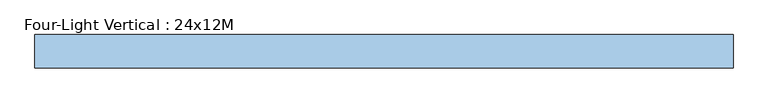
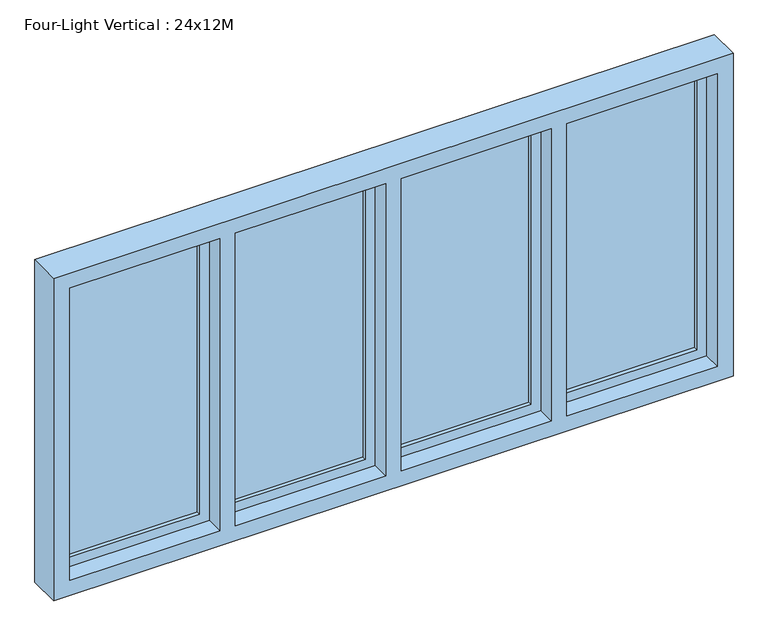
"""IFC4 building model written with IfcOpenShell, lengths in millimetres: window geometry, Four-Light Vertical : 24x12M."""

import ifcopenshell
import ifcopenshell.guid

model = None  # the IFC model being written
_history = None  # IfcOwnerHistory: only IFC2X3 demands one
_inside = {}  # id of a spatial element -> (the spatial element, [elements in it])
_under = {}  # id of a project, library or spatial element -> (it, [spatial elements below it])
_declared = {}  # id of a project -> (the project, [libraries it declares])
_typed = {}  # id of a type object -> (the type object, [elements of that type])
_made_of = {}  # id of a material, layer set ... -> (it, [elements and type objects made of it])


def new_model(schema):
    """Start an empty IFC model of exactly this schema.

    Asked for "IFC4X3", IfcOpenShell would pick the latest addendum, in which some entities
    have other attributes; the version numbers below select the first issue.
    IFC2X3 requires an IfcOwnerHistory on every rooted entity: one is made here for all.
    """
    global model, _history
    if schema == "IFC4X3":
        model = ifcopenshell.file(schema_version=(4, 3, 0, 0))
    else:
        model = ifcopenshell.file(schema=schema)
    _inside.clear()
    _under.clear()
    _declared.clear()
    _typed.clear()
    _made_of.clear()
    _history = None
    if model.schema == "IFC2X3":
        org = make("IfcOrganization", Name="unknown")
        user = make(
            "IfcPersonAndOrganization",
            ThePerson=make("IfcPerson", FamilyName="unknown"),
            TheOrganization=org,
        )
        app = make(
            "IfcApplication",
            ApplicationDeveloper=org,
            Version="unknown",
            ApplicationFullName="unknown",
            ApplicationIdentifier="unknown",
        )
        _history = make(
            "IfcOwnerHistory",
            OwningUser=user,
            OwningApplication=app,
            ChangeAction="ADDED",
            CreationDate=0,
        )
    return model


def make(cls, **values):
    """One entity of the class cls with the attributes given. An attribute that is None is left unset."""
    return model.create_entity(
        cls, **{name: value for name, value in values.items() if value is not None}
    )


def rooted(cls, **values):
    """An entity with a GlobalId (a new one), such as an element, a storey or a relation."""
    return make(cls, GlobalId=ifcopenshell.guid.new(), OwnerHistory=_history, **values)


def si_unit(unit_type, name, prefix=None):
    """IfcSIUnit, for example si_unit("LENGTHUNIT", "METRE", prefix="MILLI")."""
    return make("IfcSIUnit", UnitType=unit_type, Prefix=prefix, Name=name)


def assignment(units):
    """IfcUnitAssignment: the units of a project."""
    return None if units is None else make("IfcUnitAssignment", Units=units)


def point(xyz):
    """IfcCartesianPoint."""
    return None if xyz is None else make("IfcCartesianPoint", Coordinates=xyz)


def direction(xyz):
    """IfcDirection."""
    return None if xyz is None else make("IfcDirection", DirectionRatios=xyz)


def frame(location, z_axis=None, x_axis=None):
    """IfcAxis2Placement3D, a coordinate frame: its origin and axes. An axis left out is left unset."""
    return make(
        "IfcAxis2Placement3D",
        Location=point(location),
        Axis=direction(z_axis),
        RefDirection=direction(x_axis),
    )


def origin():
    """The frame at (0, 0, 0) with its axes left unset."""
    return frame((0.0, 0.0, 0.0))


def place(relative_to, where):
    """IfcLocalPlacement: puts the frame where relative to a parent placement (None: the world)."""
    return make(
        "IfcLocalPlacement", PlacementRelTo=relative_to, RelativePlacement=where
    )


def context(
    kind, dimensions, precision=None, world=None, true_north=None, identifier=None
):
    """IfcGeometricRepresentationContext, for example the 3D "Model" context."""
    return make(
        "IfcGeometricRepresentationContext",
        ContextIdentifier=identifier,
        ContextType=kind,
        CoordinateSpaceDimension=dimensions,
        Precision=precision,
        WorldCoordinateSystem=world,
        TrueNorth=true_north,
    )


def project(units=None, contexts=None):
    """IfcProject with its units and contexts."""
    return rooted(
        "IfcProject",
        Name="project",
        RepresentationContexts=contexts,
        UnitsInContext=assignment(units),
    )


def spatial(cls, under=None, at=None, **own):
    """A site, building, storey or space (cls), placed at a placement, below another one or the project."""
    s = rooted(cls, ObjectPlacement=at, **own)
    if under is not None:
        _under.setdefault(under.id(), (under, []))[1].append(s)
    return s


def polyline(points):
    """IfcPolyline through the points."""
    return make("IfcPolyline", Points=[point(p) for p in points])


def outline(outer, holes=None, kind="AREA"):
    """IfcArbitraryClosedProfileDef: a profile drawn as a closed curve; with holes, ...WithVoids."""
    if holes is None:
        return make("IfcArbitraryClosedProfileDef", ProfileType=kind, OuterCurve=outer)
    return make(
        "IfcArbitraryProfileDefWithVoids",
        ProfileType=kind,
        OuterCurve=outer,
        InnerCurves=holes,
    )


def extrude(swept, where, along, depth):
    """IfcExtrudedAreaSolid: the profile swept, set in the frame where, extruded along a direction by depth."""
    return make(
        "IfcExtrudedAreaSolid",
        SweptArea=swept,
        Position=where,
        ExtrudedDirection=direction(along),
        Depth=depth,
    )


def faces_of(points, faces, orient=None, outer=None):
    """IfcFace entities. A face is a list of loops; a loop is a list of indices into points, from 0.

    orient and outer hold one flag for each loop. By default every Orientation is true, the
    first loop of a face is its IfcFaceOuterBound and the others are IfcFaceBound.
    """
    made = []
    for i, loops in enumerate(faces):
        bounds = []
        for j, loop in enumerate(loops):
            is_outer = j == 0 if outer is None else outer[i][j]
            bounds.append(
                make(
                    "IfcFaceOuterBound" if is_outer else "IfcFaceBound",
                    Bound=make("IfcPolyLoop", Polygon=[points[k] for k in loop]),
                    Orientation=True if orient is None else orient[i][j],
                )
            )
        made.append(make("IfcFace", Bounds=bounds))
    return made


def faceted_brep(points, faces, orient=None, outer=None, voids=None):
    """IfcFacetedBrep: a solid bounded by flat faces; with voids (closed shells), ...WithVoids."""
    shared = [point(p) for p in points]
    hull = make("IfcClosedShell", CfsFaces=faces_of(shared, faces, orient, outer))
    if voids is None:
        return make("IfcFacetedBrep", Outer=hull)
    return make(
        "IfcFacetedBrepWithVoids",
        Outer=hull,
        Voids=[
            make(cls, CfsFaces=faces_of(shared, fs, o, b)) for cls, fs, o, b in voids
        ],
    )


def shape(context_of_items, identifier, shape_type, items):
    """IfcShapeRepresentation: the items that make up one representation, for example the "Body"."""
    return make(
        "IfcShapeRepresentation",
        ContextOfItems=context_of_items,
        RepresentationIdentifier=identifier,
        RepresentationType=shape_type,
        Items=items,
    )


def source(mapping_origin, context_of_items, identifier, shape_type, items):
    """IfcRepresentationMap: a shape defined once, which mapped items show again and again."""
    return make(
        "IfcRepresentationMap",
        MappingOrigin=mapping_origin,
        MappedRepresentation=shape(context_of_items, identifier, shape_type, items),
    )


def transform(
    local_origin,
    x_axis=None,
    y_axis=None,
    z_axis=None,
    scale=None,
    scale2=None,
    scale3=None,
    uniform=True,
):
    """IfcCartesianTransformationOperator3D, or its non-uniform kind. x_axis, y_axis, z_axis: its Axis1, 2, 3."""
    if uniform:
        return make(
            "IfcCartesianTransformationOperator3D",
            Axis1=direction(x_axis),
            Axis2=direction(y_axis),
            LocalOrigin=point(local_origin),
            Scale=scale,
            Axis3=direction(z_axis),
        )
    return make(
        "IfcCartesianTransformationOperator3DnonUniform",
        Axis1=direction(x_axis),
        Axis2=direction(y_axis),
        LocalOrigin=point(local_origin),
        Scale=scale,
        Axis3=direction(z_axis),
        Scale2=scale2,
        Scale3=scale3,
    )


def mapped(mapping_source, mapping_target):
    """IfcMappedItem: shows the shape of a source again, moved by a transform."""
    return make(
        "IfcMappedItem", MappingSource=mapping_source, MappingTarget=mapping_target
    )


def made_of(thing, what):
    """Note that an element or type object is made of a material, layer set ...; save() writes the relation."""
    if what is not None:
        _made_of.setdefault(what.id(), (what, []))[1].append(thing)
    return thing


def element(
    cls,
    number,
    at=None,
    inside=None,
    cuts=None,
    type_object=None,
    material=None,
    context=None,
    identifier="Body",
    shape_type=None,
    held_by="IfcProductDefinitionShape",
    body=None,
    shapes=None,
    **own,
):
    """One element of the class cls, such as IfcWall. Its Tag is "e" and its number.

    at: its placement. inside: the storey or other place that contains it. cuts: it is an
    opening in that element (IfcRelVoidsElement). A single representation is given by context,
    identifier, shape_type and body (its items); several are given by shapes. held_by: the class
    of the entity that holds the representations. save() writes the other relations.
    """
    e = rooted(cls, Tag="e%d" % number, ObjectPlacement=at, **own)
    if body is not None:
        shapes = [shape(context, identifier, shape_type, body)]
    if shapes is not None:
        e.Representation = make(held_by, Representations=shapes)
    if inside is not None:
        _inside.setdefault(inside.id(), (inside, []))[1].append(e)
    if cuts is not None:
        rooted(
            "IfcRelVoidsElement", RelatingBuildingElement=cuts, RelatedOpeningElement=e
        )
    if type_object is not None:
        _typed.setdefault(type_object.id(), (type_object, []))[1].append(e)
    return made_of(e, material)


def aggregate(whole, parts):
    """IfcRelAggregates: a whole, such as a stair, and the parts it consists of."""
    return rooted("IfcRelAggregates", RelatingObject=whole, RelatedObjects=parts)


def save(model, path):
    """Write the relations noted so far, then the file.

    IfcRelAggregates (storeys below a building ...), IfcRelContainedInSpatialStructure (elements
    in a storey), IfcRelDefinesByType, IfcRelAssociatesMaterial and IfcRelDeclares: one each for
    every whole, place, type object, material and project.
    """
    for whole, parts in _under.values():
        aggregate(whole, parts)
    for where, things in _inside.values():
        rooted(
            "IfcRelContainedInSpatialStructure",
            RelatedElements=things,
            RelatingStructure=where,
        )
    for kind, things in _typed.values():
        rooted("IfcRelDefinesByType", RelatedObjects=things, RelatingType=kind)
    for what, things in _made_of.values():
        rooted("IfcRelAssociatesMaterial", RelatedObjects=things, RelatingMaterial=what)
    for by, libraries in _declared.values():
        rooted("IfcRelDeclares", RelatingContext=by, RelatedDefinitions=libraries)
    model.write(path)


def four_light_vertical_24x12m_47221696(model_context):
    return source(origin(), model_context, "Body", "SolidModel", [
        extrude(outline(polyline([(1970.0, -1224.0), (842.0, -1224.0), (842.0, -660.75), (1970.0, -660.75), (1970.0, -1224.0)]), holes=[polyline([(1920.0, -710.75), (892.0, -710.75), (892.0, -1174.0), (1920.0, -1174.0), (1920.0, -710.75)])]), frame((0.0, 134.0, 0.0), z_axis=(0.0, 1.0, 0.0), x_axis=(0.0, 0.0, 1.0)), (0.0, 0.0, 1.0), 50.0),
        extrude(outline(polyline([(1970.0, -635.75), (842.0, -635.75), (842.0, -72.5), (1970.0, -72.5), (1970.0, -635.75)]), holes=[polyline([(1920.0, -122.5), (892.0, -122.5), (892.0, -585.75), (1920.0, -585.75), (1920.0, -122.5)])]), frame((0.0, 134.0, 0.0), z_axis=(0.0, 1.0, 0.0), x_axis=(0.0, 0.0, 1.0)), (0.0, 0.0, 1.0), 50.0),
        extrude(outline(polyline([(1970.0, -47.5), (842.0, -47.5), (842.0, 515.75), (1970.0, 515.75), (1970.0, -47.5)]), holes=[polyline([(1920.0, 465.75), (892.0, 465.75), (892.0, 2.5), (1920.0, 2.5), (1920.0, 465.75)])]), frame((0.0, 134.0, 0.0), z_axis=(0.0, 1.0, 0.0), x_axis=(0.0, 0.0, 1.0)), (0.0, 0.0, 1.0), 50.0),
        extrude(outline(polyline([(1970.0, 540.75), (842.0, 540.75), (842.0, 1104.0), (1970.0, 1104.0), (1970.0, 540.75)]), holes=[polyline([(1920.0, 1054.0), (892.0, 1054.0), (892.0, 590.75), (1920.0, 590.75), (1920.0, 1054.0)])]), frame((0.0, 134.0, 0.0), z_axis=(0.0, 1.0, 0.0), x_axis=(0.0, 0.0, 1.0)), (0.0, 0.0, 1.0), 50.0),
        faceted_brep([(-1266.0, 184.0, 800.0), (1146.0, 184.0, 800.0), (1146.0, 69.0, 800.0), (-1266.0, 69.0, 800.0), (1146.0, 184.0, 2012.0), (1146.0, 69.0, 2012.0), (-1266.0, 184.0, 2012.0), (1104.0, 184.0, 842.0), (1104.0, 184.0, 1970.0), (540.75, 184.0, 1970.0), (540.75, 184.0, 842.0), (-1224.0, 184.0, 1970.0), (-1224.0, 184.0, 842.0), (-660.75, 184.0, 842.0), (-660.75, 184.0, 1970.0), (515.75, 184.0, 842.0), (515.75, 184.0, 1970.0), (-47.5, 184.0, 1970.0), (-47.5, 184.0, 842.0), (-72.5, 184.0, 1970.0), (-635.75, 184.0, 1970.0), (-635.75, 184.0, 842.0), (-72.5, 184.0, 842.0), (-1266.0, 69.0, 2012.0), (1089.0, 69.0, 1955.0), (1089.0, 69.0, 857.0), (555.75, 69.0, 857.0), (555.75, 69.0, 1955.0), (500.75, 69.0, 1955.0), (500.75, 69.0, 857.0), (-32.5, 69.0, 857.0), (-32.5, 69.0, 1955.0), (-87.5, 69.0, 857.0), (-620.75, 69.0, 857.0), (-620.75, 69.0, 1955.0), (-87.5, 69.0, 1955.0), (-1209.0, 69.0, 857.0), (-1209.0, 69.0, 1955.0), (-675.75, 69.0, 1955.0), (-675.75, 69.0, 857.0), (1089.0, 134.0, 857.0), (555.75, 134.0, 857.0), (-1209.0, 134.0, 857.0), (-675.75, 134.0, 857.0), (500.75, 134.0, 857.0), (-32.5, 134.0, 857.0), (-87.5, 134.0, 857.0), (-620.75, 134.0, 857.0), (1089.0, 134.0, 1955.0), (1104.0, 134.0, 1970.0), (1104.0, 134.0, 842.0), (540.75, 134.0, 842.0), (540.75, 134.0, 1970.0), (555.75, 134.0, 1955.0), (-1224.0, 134.0, 842.0), (-1224.0, 134.0, 1970.0), (-660.75, 134.0, 1970.0), (-660.75, 134.0, 842.0), (-1209.0, 134.0, 1955.0), (-675.75, 134.0, 1955.0), (515.75, 134.0, 1970.0), (515.75, 134.0, 842.0), (-47.5, 134.0, 842.0), (-47.5, 134.0, 1970.0), (500.75, 134.0, 1955.0), (-32.5, 134.0, 1955.0), (-72.5, 134.0, 1970.0), (-72.5, 134.0, 842.0), (-635.75, 134.0, 842.0), (-635.75, 134.0, 1970.0), (-87.5, 134.0, 1955.0), (-620.75, 134.0, 1955.0)], [[[0, 1, 2, 3]], [[2, 1, 4, 5]], [[4, 1, 0, 6], [7, 8, 9, 10], [11, 12, 13, 14], [15, 16, 17, 18], [19, 20, 21, 22]], [[2, 5, 23, 3], [24, 25, 26, 27], [28, 29, 30, 31], [32, 33, 34, 35], [36, 37, 38, 39]], [[25, 40, 41, 26]], [[42, 36, 39, 43]], [[29, 44, 45, 30]], [[32, 46, 47, 33]], [[40, 25, 24, 48]], [[49, 50, 51, 52], [40, 48, 53, 41]], [[54, 55, 56, 57], [58, 42, 43, 59]], [[60, 61, 62, 63], [44, 64, 65, 45]], [[66, 67, 68, 69], [46, 70, 71, 47]], [[68, 67, 22, 21]], [[50, 7, 10, 51]], [[12, 54, 57, 13]], [[61, 15, 18, 62]], [[7, 50, 49, 8]], [[23, 6, 0, 3]], [[58, 37, 36, 42]], [[11, 55, 54, 12]], [[10, 9, 52, 51]], [[27, 26, 41, 53]], [[29, 28, 64, 44]], [[16, 15, 61, 60]], [[18, 17, 63, 62]], [[31, 30, 45, 65]], [[32, 35, 70, 46]], [[19, 22, 67, 66]], [[21, 20, 69, 68]], [[34, 33, 47, 71]], [[39, 38, 59, 43]], [[14, 13, 57, 56]], [[23, 5, 4, 6]], [[48, 24, 27, 53]], [[37, 58, 59, 38]], [[64, 28, 31, 65]], [[70, 35, 34, 71]], [[8, 49, 52, 9]], [[16, 60, 63, 17]], [[19, 66, 69, 20]], [[56, 55, 11, 14]]]),
        extrude(outline(polyline([(2.5, 170.0), (465.75, 170.0), (465.75, 148.0), (2.5, 148.0), (2.5, 170.0)])), frame((0.0, 0.0, 892.0), z_axis=(0.0, 0.0, 1.0), x_axis=(1.0, 0.0, 0.0)), (0.0, 0.0, 1.0), 1028.0),
        extrude(outline(polyline([(-585.75, 170.0), (-122.5, 170.0), (-122.5, 148.0), (-585.75, 148.0), (-585.75, 170.0)])), frame((0.0, 0.0, 892.0), z_axis=(0.0, 0.0, 1.0), x_axis=(1.0, 0.0, 0.0)), (0.0, 0.0, 1.0), 1028.0),
        extrude(outline(polyline([(-1174.0, 170.0), (-710.75, 170.0), (-710.75, 148.0), (-1174.0, 148.0), (-1174.0, 170.0)])), frame((0.0, 0.0, 892.0), z_axis=(0.0, 0.0, 1.0), x_axis=(1.0, 0.0, 0.0)), (0.0, 0.0, 1.0), 1028.0),
        extrude(outline(polyline([(590.75, 170.0), (1054.0, 170.0), (1054.0, 148.0), (590.75, 148.0), (590.75, 170.0)])), frame((0.0, 0.0, 892.0), z_axis=(0.0, 0.0, 1.0), x_axis=(1.0, 0.0, 0.0)), (0.0, 0.0, 1.0), 1028.0),
    ])


if __name__ == "__main__":
    model = new_model("IFC4")
    model_context = context("Model", 3, world=origin())
    ifc_project = project(units=[si_unit("LENGTHUNIT", "METRE", prefix="MILLI")], contexts=[model_context])
    site = spatial("IfcSite", under=ifc_project)
    building = spatial("IfcBuilding", under=site)
    placement = place(None, origin())
    four_light_vertical_24x12m_shape = four_light_vertical_24x12m_47221696(model_context)
    element("IfcWindow", 1, ObjectType="Four-Light Vertical : 24x12M", at=placement, inside=building, context=model_context, shape_type="MappedRepresentation", body=[
        mapped(four_light_vertical_24x12m_shape, transform((0.0, 0.0, 0.0), x_axis=(1.0, 0.0, 0.0), y_axis=(0.0, 1.0, 0.0), z_axis=(0.0, 0.0, 1.0))),
    ])
    save(model, "model.ifc")

# Revit data of these elements
# Type "Four-Light Vertical : 24x12M"
#   Type Mark = "53"
#   Creator Organization [instance default] = "© Danish Educational Content"
#   Creator Name [instance default] = "© Erik Falck Jørgensen"
#   Creator Build [instance default] = "2017.0801.0"
#   Analytic Construction = "<None>"
#   length#6 = -36 mm
#   length#5 = -14 mm
#   length#3 = 29.5 mm
#   length#2 = 57 mm
#   length#1 = 0 mm
#   length#4 = 120 mm
#   Seal Width = 12 mm
#   Rough Width = 2412 mm
#   Rough Height = 1212 mm
#   Rebate Depth = 50 mm
#   Transom Width = 55 mm
#   Rabbet Width = 15 mm
#   Rabbet Depth = 50 mm
#   Height = 1188 mm
#   Glass Thickness = 22 mm
#   Frame Width = 50 mm
#   Frame Depth = 50 mm
#   Exterior Direction [instance default] = 0.00°
#   Case Depth = 115 mm
#   Case Width = 45 mm
#   Default Sill Height = 800 mm
#   Width = 2388 mm
#   Sealing = no
#   Hinging = yes
#   Wall Closure = 1
#   Above Cutplane [instance default] = no
#   Glass = none
#   Case/Transom = none
#   Frame/Mullion = none
#   Assembly Code = ""
# Element 1 (IfcWindow, "Four-Light Vertical : 24x12M")
#   Materials on its faces: "Default Frame/Mullion (Interior/Exterior)", "Glass"
# Materials
#   "Default Frame/Mullion (Interior/Exterior)": class "Generic", colour RGB 205 205 205, transparency 0, Description = "Udefineret karm/ramme materiale", Cost = 0
#   "Glass": class "Glass", colour RGB 180 200 255, transparency 0.75, Description = "Generisk glas", Cost = 0
